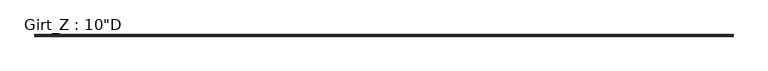
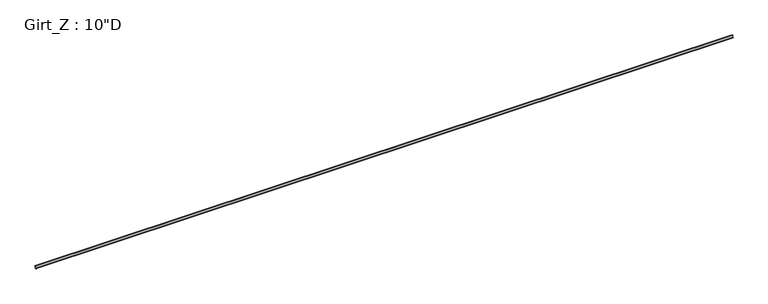
"""IFC4 building model written with IfcOpenShell, lengths in millimetres: beam geometry."""

from ifc_helpers import new_model, si_unit, point, frame, frame_2d, origin, place, context, project, spatial, polyline, circle_curve, trimmed, segment, composite_curve, outline, extrude, source, transform, mapped, element, save


def beam_9902b02c(model_context):
    return source(origin(), model_context, "Body", "SweptSolid", [
        extrude(outline(composite_curve([segment(polyline([(77.9859375, 127.0), (90.2310415, 112.4068534), (88.1028742, 110.621109), (76.6904765, 124.221875), (3.3005807, 124.221875)]), True, "CONTINUOUS"), segment(trimmed(circle_curve(frame_2d((3.3741066, 122.2381931)), 1.9850441), [point((3.3005807, 124.221875))], [point((1.3890625, 122.2381931))], True, "CARTESIAN"), True, "CONTINUOUS"), segment(polyline([(1.3890625, 122.2381931), (1.3890625, -127.0), (-84.3359375, -127.0), (-96.5810415, -112.4068534), (-94.4528742, -110.621109), (-83.0404765, -124.221875), (-3.2694106, -124.221875)]), True, "CONTINUOUS"), segment(trimmed(circle_curve(frame_2d((-3.3748024, -122.2389339)), 1.9857399), [point((-3.2694106, -124.221875))], [point((-1.3890625, -122.2389339))], True, "CARTESIAN"), True, "CONTINUOUS"), segment(polyline([(-1.3890625, -122.2389339), (-1.3890625, 122.2375)]), True, "CONTINUOUS"), segment(trimmed(circle_curve(frame_2d((3.3734375, 122.2375)), 4.7625), [point((-1.3890625, 122.2375))], [point((3.3734375, 127.0))], False, "CARTESIAN"), True, "CONTINUOUS"), segment(polyline([(3.3734375, 127.0), (77.9859375, 127.0)]), True, "CONTINUOUS")], self_intersect=False)), frame((-40536.4315, 0.0, 0.0), z_axis=(1.0, 0.0, 0.0), x_axis=(0.0, 1.0, 0.0)), (0.0, 0.0, 1.0), 81158.969),
    ])


if __name__ == "__main__":
    model = new_model("IFC4")
    model_context = context("Model", 3, world=origin())
    ifc_project = project(units=[si_unit("LENGTHUNIT", "METRE", prefix="MILLI")], contexts=[model_context])
    site = spatial("IfcSite", under=ifc_project)
    building = spatial("IfcBuilding", under=site)
    placement = place(None, origin())
    beam_shape = beam_9902b02c(model_context)
    element("IfcBeam", 1, ObjectType="Girt_Z : 10\"D", at=placement, inside=building, context=model_context, shape_type="MappedRepresentation", body=[
        mapped(beam_shape, transform((0.0, 0.0, 0.0), x_axis=(1.0, 0.0, 0.0), y_axis=(0.0, 1.0, 0.0), z_axis=(0.0, 0.0, 1.0))),
    ])
    save(model, "model.ifc")

# Revit data of these elements
# Type "Girt_Z : 10\"D"
#   half leg = 0' - 1 11/16"
#   Web_Thickness = 0' - 0 7/64"
#   Length [instance default] = 10' - 0"
#   Leg_2 = 0' - 3 3/8"
#   Leg_1 = 0' - 3 1/8"
#   Height = 0' - 10"
#   Structural Material [instance default] = none
# Element 1 (IfcBeam, "Girt_Z : 10\"D")
#   Materials on its faces: "STRUCTURAL STEEL - SEE STRUCT. DWGS"
# Materials
#   "STRUCTURAL STEEL - SEE STRUCT. DWGS": class "Metal", colour RGB 137 146 153, transparency 0, Description = "Steel, mill finish", Cost = 0
